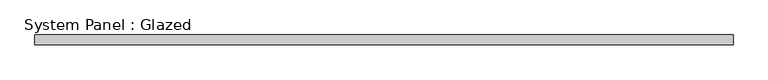
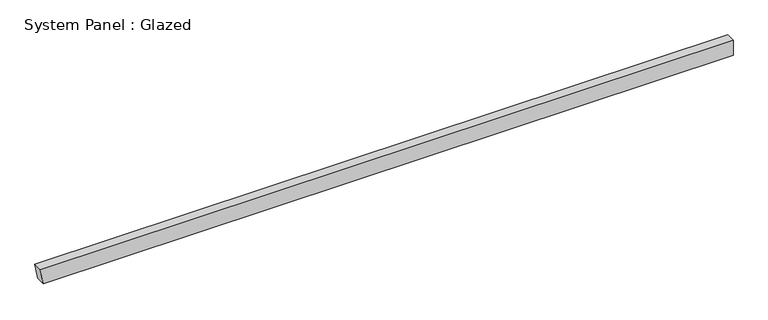
"""IFC4 building model written with IfcOpenShell, lengths in millimetres: plate geometry, System Panel : Glazed."""

import ifcopenshell
import ifcopenshell.guid

model = None  # the IFC model being written
_history = None  # IfcOwnerHistory: only IFC2X3 demands one
_inside = {}  # id of a spatial element -> (the spatial element, [elements in it])
_under = {}  # id of a project, library or spatial element -> (it, [spatial elements below it])
_declared = {}  # id of a project -> (the project, [libraries it declares])
_typed = {}  # id of a type object -> (the type object, [elements of that type])
_made_of = {}  # id of a material, layer set ... -> (it, [elements and type objects made of it])


def new_model(schema):
    """Start an empty IFC model of exactly this schema.

    Asked for "IFC4X3", IfcOpenShell would pick the latest addendum, in which some entities
    have other attributes; the version numbers below select the first issue.
    IFC2X3 requires an IfcOwnerHistory on every rooted entity: one is made here for all.
    """
    global model, _history
    if schema == "IFC4X3":
        model = ifcopenshell.file(schema_version=(4, 3, 0, 0))
    else:
        model = ifcopenshell.file(schema=schema)
    _inside.clear()
    _under.clear()
    _declared.clear()
    _typed.clear()
    _made_of.clear()
    _history = None
    if model.schema == "IFC2X3":
        org = make("IfcOrganization", Name="unknown")
        user = make(
            "IfcPersonAndOrganization",
            ThePerson=make("IfcPerson", FamilyName="unknown"),
            TheOrganization=org,
        )
        app = make(
            "IfcApplication",
            ApplicationDeveloper=org,
            Version="unknown",
            ApplicationFullName="unknown",
            ApplicationIdentifier="unknown",
        )
        _history = make(
            "IfcOwnerHistory",
            OwningUser=user,
            OwningApplication=app,
            ChangeAction="ADDED",
            CreationDate=0,
        )
    return model


def make(cls, **values):
    """One entity of the class cls with the attributes given. An attribute that is None is left unset."""
    return model.create_entity(
        cls, **{name: value for name, value in values.items() if value is not None}
    )


def rooted(cls, **values):
    """An entity with a GlobalId (a new one), such as an element, a storey or a relation."""
    return make(cls, GlobalId=ifcopenshell.guid.new(), OwnerHistory=_history, **values)


def si_unit(unit_type, name, prefix=None):
    """IfcSIUnit, for example si_unit("LENGTHUNIT", "METRE", prefix="MILLI")."""
    return make("IfcSIUnit", UnitType=unit_type, Prefix=prefix, Name=name)


def assignment(units):
    """IfcUnitAssignment: the units of a project."""
    return None if units is None else make("IfcUnitAssignment", Units=units)


def point(xyz):
    """IfcCartesianPoint."""
    return None if xyz is None else make("IfcCartesianPoint", Coordinates=xyz)


def direction(xyz):
    """IfcDirection."""
    return None if xyz is None else make("IfcDirection", DirectionRatios=xyz)


def frame(location, z_axis=None, x_axis=None):
    """IfcAxis2Placement3D, a coordinate frame: its origin and axes. An axis left out is left unset."""
    return make(
        "IfcAxis2Placement3D",
        Location=point(location),
        Axis=direction(z_axis),
        RefDirection=direction(x_axis),
    )


def origin():
    """The frame at (0, 0, 0) with its axes left unset."""
    return frame((0.0, 0.0, 0.0))


def place(relative_to, where):
    """IfcLocalPlacement: puts the frame where relative to a parent placement (None: the world)."""
    return make(
        "IfcLocalPlacement", PlacementRelTo=relative_to, RelativePlacement=where
    )


def context(
    kind, dimensions, precision=None, world=None, true_north=None, identifier=None
):
    """IfcGeometricRepresentationContext, for example the 3D "Model" context."""
    return make(
        "IfcGeometricRepresentationContext",
        ContextIdentifier=identifier,
        ContextType=kind,
        CoordinateSpaceDimension=dimensions,
        Precision=precision,
        WorldCoordinateSystem=world,
        TrueNorth=true_north,
    )


def project(units=None, contexts=None):
    """IfcProject with its units and contexts."""
    return rooted(
        "IfcProject",
        Name="project",
        RepresentationContexts=contexts,
        UnitsInContext=assignment(units),
    )


def spatial(cls, under=None, at=None, **own):
    """A site, building, storey or space (cls), placed at a placement, below another one or the project."""
    s = rooted(cls, ObjectPlacement=at, **own)
    if under is not None:
        _under.setdefault(under.id(), (under, []))[1].append(s)
    return s


def polyline(points):
    """IfcPolyline through the points."""
    return make("IfcPolyline", Points=[point(p) for p in points])


def outline(outer, holes=None, kind="AREA"):
    """IfcArbitraryClosedProfileDef: a profile drawn as a closed curve; with holes, ...WithVoids."""
    if holes is None:
        return make("IfcArbitraryClosedProfileDef", ProfileType=kind, OuterCurve=outer)
    return make(
        "IfcArbitraryProfileDefWithVoids",
        ProfileType=kind,
        OuterCurve=outer,
        InnerCurves=holes,
    )


def extrude(swept, where, along, depth):
    """IfcExtrudedAreaSolid: the profile swept, set in the frame where, extruded along a direction by depth."""
    return make(
        "IfcExtrudedAreaSolid",
        SweptArea=swept,
        Position=where,
        ExtrudedDirection=direction(along),
        Depth=depth,
    )


def shape(context_of_items, identifier, shape_type, items):
    """IfcShapeRepresentation: the items that make up one representation, for example the "Body"."""
    return make(
        "IfcShapeRepresentation",
        ContextOfItems=context_of_items,
        RepresentationIdentifier=identifier,
        RepresentationType=shape_type,
        Items=items,
    )


def source(mapping_origin, context_of_items, identifier, shape_type, items):
    """IfcRepresentationMap: a shape defined once, which mapped items show again and again."""
    return make(
        "IfcRepresentationMap",
        MappingOrigin=mapping_origin,
        MappedRepresentation=shape(context_of_items, identifier, shape_type, items),
    )


def transform(
    local_origin,
    x_axis=None,
    y_axis=None,
    z_axis=None,
    scale=None,
    scale2=None,
    scale3=None,
    uniform=True,
):
    """IfcCartesianTransformationOperator3D, or its non-uniform kind. x_axis, y_axis, z_axis: its Axis1, 2, 3."""
    if uniform:
        return make(
            "IfcCartesianTransformationOperator3D",
            Axis1=direction(x_axis),
            Axis2=direction(y_axis),
            LocalOrigin=point(local_origin),
            Scale=scale,
            Axis3=direction(z_axis),
        )
    return make(
        "IfcCartesianTransformationOperator3DnonUniform",
        Axis1=direction(x_axis),
        Axis2=direction(y_axis),
        LocalOrigin=point(local_origin),
        Scale=scale,
        Axis3=direction(z_axis),
        Scale2=scale2,
        Scale3=scale3,
    )


def mapped(mapping_source, mapping_target):
    """IfcMappedItem: shows the shape of a source again, moved by a transform."""
    return make(
        "IfcMappedItem", MappingSource=mapping_source, MappingTarget=mapping_target
    )


def made_of(thing, what):
    """Note that an element or type object is made of a material, layer set ...; save() writes the relation."""
    if what is not None:
        _made_of.setdefault(what.id(), (what, []))[1].append(thing)
    return thing


def element(
    cls,
    number,
    at=None,
    inside=None,
    cuts=None,
    type_object=None,
    material=None,
    context=None,
    identifier="Body",
    shape_type=None,
    held_by="IfcProductDefinitionShape",
    body=None,
    shapes=None,
    **own,
):
    """One element of the class cls, such as IfcWall. Its Tag is "e" and its number.

    at: its placement. inside: the storey or other place that contains it. cuts: it is an
    opening in that element (IfcRelVoidsElement). A single representation is given by context,
    identifier, shape_type and body (its items); several are given by shapes. held_by: the class
    of the entity that holds the representations. save() writes the other relations.
    """
    e = rooted(cls, Tag="e%d" % number, ObjectPlacement=at, **own)
    if body is not None:
        shapes = [shape(context, identifier, shape_type, body)]
    if shapes is not None:
        e.Representation = make(held_by, Representations=shapes)
    if inside is not None:
        _inside.setdefault(inside.id(), (inside, []))[1].append(e)
    if cuts is not None:
        rooted(
            "IfcRelVoidsElement", RelatingBuildingElement=cuts, RelatedOpeningElement=e
        )
    if type_object is not None:
        _typed.setdefault(type_object.id(), (type_object, []))[1].append(e)
    return made_of(e, material)


def aggregate(whole, parts):
    """IfcRelAggregates: a whole, such as a stair, and the parts it consists of."""
    return rooted("IfcRelAggregates", RelatingObject=whole, RelatedObjects=parts)


def save(model, path):
    """Write the relations noted so far, then the file.

    IfcRelAggregates (storeys below a building ...), IfcRelContainedInSpatialStructure (elements
    in a storey), IfcRelDefinesByType, IfcRelAssociatesMaterial and IfcRelDeclares: one each for
    every whole, place, type object, material and project.
    """
    for whole, parts in _under.values():
        aggregate(whole, parts)
    for where, things in _inside.values():
        rooted(
            "IfcRelContainedInSpatialStructure",
            RelatedElements=things,
            RelatingStructure=where,
        )
    for kind, things in _typed.values():
        rooted("IfcRelDefinesByType", RelatedObjects=things, RelatingType=kind)
    for what, things in _made_of.values():
        rooted("IfcRelAssociatesMaterial", RelatedObjects=things, RelatingMaterial=what)
    for by, libraries in _declared.values():
        rooted("IfcRelDeclares", RelatingContext=by, RelatedDefinitions=libraries)
    model.write(path)


def system_panel_glazed_0a43eb3e(model_context):
    return source(origin(), model_context, "Body", "SweptSolid", [
        extrude(outline(polyline([(0.0, -907.0374994), (0.0, 914.4000002), (41.9143134, 914.4000002), (41.9143134, -914.4000002), (0.0, -907.0374994)])), frame((0.0, -44.45, 0.0), z_axis=(0.0, 1.0, 0.0), x_axis=(0.0, 0.0, 1.0)), (0.0, 0.0, 1.0), 25.4),
    ])


if __name__ == "__main__":
    model = new_model("IFC4")
    model_context = context("Model", 3, world=origin())
    ifc_project = project(units=[si_unit("LENGTHUNIT", "METRE", prefix="MILLI")], contexts=[model_context])
    site = spatial("IfcSite", under=ifc_project)
    building = spatial("IfcBuilding", under=site)
    placement = place(None, origin())
    system_panel_glazed_shape = system_panel_glazed_0a43eb3e(model_context)
    element("IfcPlate", 1, ObjectType="System Panel : Glazed", at=placement, inside=building, context=model_context, shape_type="MappedRepresentation", body=[
        mapped(system_panel_glazed_shape, transform((0.0, 0.0, 0.0), x_axis=(1.0, 0.0, 0.0), y_axis=(0.0, 1.0, 0.0), z_axis=(0.0, 0.0, 1.0))),
    ])
    save(model, "model.ifc")

# Revit data of these elements
# Project information
#   Organization Name = "G3B Press"
#   Organization Description = "Paul F. Aubin Cosulting Services, Inc."
#   Building Name = "Revit Essentials for Architecture"
#   Author = "Paul F. Aubin"
#   Author Website = "https://www.paulaubin.com"
#   Copyright = "Copyright © 2020 Paul F Aubin, all rights reserved"
#   Design Option = "Main Model"
#   Project Issue Date = "8/1/2020"
#   Project Status = "Design Development"
#   Client Name = "Floors and Roofs"
#   Project Address = "123 State ST\nSuite 301\nChicago, IL 60606"
#   Project Name = "09 Commercial_Complete"
#   Project Number = "2020.04A"
# Type "System Panel : Glazed"
#   Construction Type Id = "GSP4R"
#   Analytic Construction = "1/8 in Pilkington single glazing"
#   Visual Light Transmittance = 0.9
#   Solar Heat Gain Coefficient = 0.86
#   Heat Transfer Coefficient (U) = 1.18115 BTU/(h·ft²·°F)
#   Define Thermal Properties by = 1
# Element 1 (IfcPlate, "System Panel : Glazed")
#   Materials on its faces: "Glass"
# Materials
#   "Glass": class "Glass", colour RGB 0 128 192, transparency 0.75, Description = "Soda Lime Glass", Cost = 0
